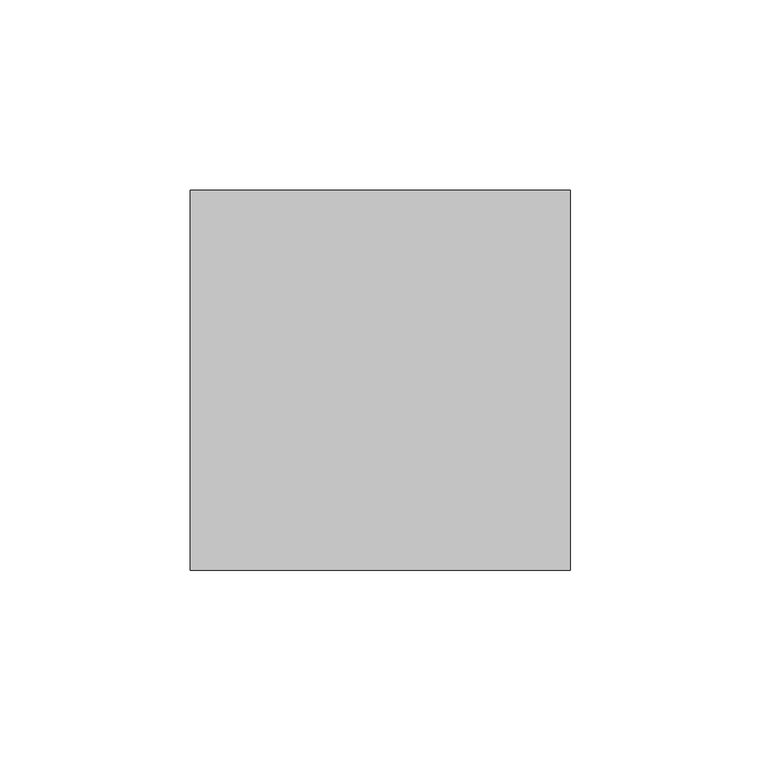
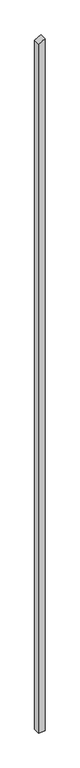
"""IFC4 building model written with IfcOpenShell, lengths in millimetres: column geometry, Holzstütze 158756 : Holzstütze 158756."""

import ifcopenshell
import ifcopenshell.guid

model = None  # the IFC model being written
_history = None  # IfcOwnerHistory: only IFC2X3 demands one
_inside = {}  # id of a spatial element -> (the spatial element, [elements in it])
_under = {}  # id of a project, library or spatial element -> (it, [spatial elements below it])
_declared = {}  # id of a project -> (the project, [libraries it declares])
_typed = {}  # id of a type object -> (the type object, [elements of that type])
_made_of = {}  # id of a material, layer set ... -> (it, [elements and type objects made of it])


def new_model(schema):
    """Start an empty IFC model of exactly this schema.

    Asked for "IFC4X3", IfcOpenShell would pick the latest addendum, in which some entities
    have other attributes; the version numbers below select the first issue.
    IFC2X3 requires an IfcOwnerHistory on every rooted entity: one is made here for all.
    """
    global model, _history
    if schema == "IFC4X3":
        model = ifcopenshell.file(schema_version=(4, 3, 0, 0))
    else:
        model = ifcopenshell.file(schema=schema)
    _inside.clear()
    _under.clear()
    _declared.clear()
    _typed.clear()
    _made_of.clear()
    _history = None
    if model.schema == "IFC2X3":
        org = make("IfcOrganization", Name="unknown")
        user = make(
            "IfcPersonAndOrganization",
            ThePerson=make("IfcPerson", FamilyName="unknown"),
            TheOrganization=org,
        )
        app = make(
            "IfcApplication",
            ApplicationDeveloper=org,
            Version="unknown",
            ApplicationFullName="unknown",
            ApplicationIdentifier="unknown",
        )
        _history = make(
            "IfcOwnerHistory",
            OwningUser=user,
            OwningApplication=app,
            ChangeAction="ADDED",
            CreationDate=0,
        )
    return model


def make(cls, **values):
    """One entity of the class cls with the attributes given. An attribute that is None is left unset."""
    return model.create_entity(
        cls, **{name: value for name, value in values.items() if value is not None}
    )


def rooted(cls, **values):
    """An entity with a GlobalId (a new one), such as an element, a storey or a relation."""
    return make(cls, GlobalId=ifcopenshell.guid.new(), OwnerHistory=_history, **values)


def si_unit(unit_type, name, prefix=None):
    """IfcSIUnit, for example si_unit("LENGTHUNIT", "METRE", prefix="MILLI")."""
    return make("IfcSIUnit", UnitType=unit_type, Prefix=prefix, Name=name)


def assignment(units):
    """IfcUnitAssignment: the units of a project."""
    return None if units is None else make("IfcUnitAssignment", Units=units)


def point(xyz):
    """IfcCartesianPoint."""
    return None if xyz is None else make("IfcCartesianPoint", Coordinates=xyz)


def direction(xyz):
    """IfcDirection."""
    return None if xyz is None else make("IfcDirection", DirectionRatios=xyz)


def frame(location, z_axis=None, x_axis=None):
    """IfcAxis2Placement3D, a coordinate frame: its origin and axes. An axis left out is left unset."""
    return make(
        "IfcAxis2Placement3D",
        Location=point(location),
        Axis=direction(z_axis),
        RefDirection=direction(x_axis),
    )


def origin():
    """The frame at (0, 0, 0) with its axes left unset."""
    return frame((0.0, 0.0, 0.0))


def place(relative_to, where):
    """IfcLocalPlacement: puts the frame where relative to a parent placement (None: the world)."""
    return make(
        "IfcLocalPlacement", PlacementRelTo=relative_to, RelativePlacement=where
    )


def context(
    kind, dimensions, precision=None, world=None, true_north=None, identifier=None
):
    """IfcGeometricRepresentationContext, for example the 3D "Model" context."""
    return make(
        "IfcGeometricRepresentationContext",
        ContextIdentifier=identifier,
        ContextType=kind,
        CoordinateSpaceDimension=dimensions,
        Precision=precision,
        WorldCoordinateSystem=world,
        TrueNorth=true_north,
    )


def project(units=None, contexts=None):
    """IfcProject with its units and contexts."""
    return rooted(
        "IfcProject",
        Name="project",
        RepresentationContexts=contexts,
        UnitsInContext=assignment(units),
    )


def spatial(cls, under=None, at=None, **own):
    """A site, building, storey or space (cls), placed at a placement, below another one or the project."""
    s = rooted(cls, ObjectPlacement=at, **own)
    if under is not None:
        _under.setdefault(under.id(), (under, []))[1].append(s)
    return s


def polyline(points):
    """IfcPolyline through the points."""
    return make("IfcPolyline", Points=[point(p) for p in points])


def outline(outer, holes=None, kind="AREA"):
    """IfcArbitraryClosedProfileDef: a profile drawn as a closed curve; with holes, ...WithVoids."""
    if holes is None:
        return make("IfcArbitraryClosedProfileDef", ProfileType=kind, OuterCurve=outer)
    return make(
        "IfcArbitraryProfileDefWithVoids",
        ProfileType=kind,
        OuterCurve=outer,
        InnerCurves=holes,
    )


def extrude(swept, where, along, depth):
    """IfcExtrudedAreaSolid: the profile swept, set in the frame where, extruded along a direction by depth."""
    return make(
        "IfcExtrudedAreaSolid",
        SweptArea=swept,
        Position=where,
        ExtrudedDirection=direction(along),
        Depth=depth,
    )


def shape(context_of_items, identifier, shape_type, items):
    """IfcShapeRepresentation: the items that make up one representation, for example the "Body"."""
    return make(
        "IfcShapeRepresentation",
        ContextOfItems=context_of_items,
        RepresentationIdentifier=identifier,
        RepresentationType=shape_type,
        Items=items,
    )


def source(mapping_origin, context_of_items, identifier, shape_type, items):
    """IfcRepresentationMap: a shape defined once, which mapped items show again and again."""
    return make(
        "IfcRepresentationMap",
        MappingOrigin=mapping_origin,
        MappedRepresentation=shape(context_of_items, identifier, shape_type, items),
    )


def transform(
    local_origin,
    x_axis=None,
    y_axis=None,
    z_axis=None,
    scale=None,
    scale2=None,
    scale3=None,
    uniform=True,
):
    """IfcCartesianTransformationOperator3D, or its non-uniform kind. x_axis, y_axis, z_axis: its Axis1, 2, 3."""
    if uniform:
        return make(
            "IfcCartesianTransformationOperator3D",
            Axis1=direction(x_axis),
            Axis2=direction(y_axis),
            LocalOrigin=point(local_origin),
            Scale=scale,
            Axis3=direction(z_axis),
        )
    return make(
        "IfcCartesianTransformationOperator3DnonUniform",
        Axis1=direction(x_axis),
        Axis2=direction(y_axis),
        LocalOrigin=point(local_origin),
        Scale=scale,
        Axis3=direction(z_axis),
        Scale2=scale2,
        Scale3=scale3,
    )


def mapped(mapping_source, mapping_target):
    """IfcMappedItem: shows the shape of a source again, moved by a transform."""
    return make(
        "IfcMappedItem", MappingSource=mapping_source, MappingTarget=mapping_target
    )


def made_of(thing, what):
    """Note that an element or type object is made of a material, layer set ...; save() writes the relation."""
    if what is not None:
        _made_of.setdefault(what.id(), (what, []))[1].append(thing)
    return thing


def element(
    cls,
    number,
    at=None,
    inside=None,
    cuts=None,
    type_object=None,
    material=None,
    context=None,
    identifier="Body",
    shape_type=None,
    held_by="IfcProductDefinitionShape",
    body=None,
    shapes=None,
    **own,
):
    """One element of the class cls, such as IfcWall. Its Tag is "e" and its number.

    at: its placement. inside: the storey or other place that contains it. cuts: it is an
    opening in that element (IfcRelVoidsElement). A single representation is given by context,
    identifier, shape_type and body (its items); several are given by shapes. held_by: the class
    of the entity that holds the representations. save() writes the other relations.
    """
    e = rooted(cls, Tag="e%d" % number, ObjectPlacement=at, **own)
    if body is not None:
        shapes = [shape(context, identifier, shape_type, body)]
    if shapes is not None:
        e.Representation = make(held_by, Representations=shapes)
    if inside is not None:
        _inside.setdefault(inside.id(), (inside, []))[1].append(e)
    if cuts is not None:
        rooted(
            "IfcRelVoidsElement", RelatingBuildingElement=cuts, RelatedOpeningElement=e
        )
    if type_object is not None:
        _typed.setdefault(type_object.id(), (type_object, []))[1].append(e)
    return made_of(e, material)


def aggregate(whole, parts):
    """IfcRelAggregates: a whole, such as a stair, and the parts it consists of."""
    return rooted("IfcRelAggregates", RelatingObject=whole, RelatedObjects=parts)


def save(model, path):
    """Write the relations noted so far, then the file.

    IfcRelAggregates (storeys below a building ...), IfcRelContainedInSpatialStructure (elements
    in a storey), IfcRelDefinesByType, IfcRelAssociatesMaterial and IfcRelDeclares: one each for
    every whole, place, type object, material and project.
    """
    for whole, parts in _under.values():
        aggregate(whole, parts)
    for where, things in _inside.values():
        rooted(
            "IfcRelContainedInSpatialStructure",
            RelatedElements=things,
            RelatingStructure=where,
        )
    for kind, things in _typed.values():
        rooted("IfcRelDefinesByType", RelatedObjects=things, RelatingType=kind)
    for what, things in _made_of.values():
        rooted("IfcRelAssociatesMaterial", RelatedObjects=things, RelatingMaterial=what)
    for by, libraries in _declared.values():
        rooted("IfcRelDeclares", RelatingContext=by, RelatedDefinitions=libraries)
    model.write(path)


def column_c7102fa8(model_context):
    return source(origin(), model_context, "Body", "SweptSolid", [
        extrude(outline(polyline([(-500.0, 165627.7593015), (-500.0, 165727.7593015), (10641.011365, 165727.7593015), (10590.0588201, 165627.7593015), (-500.0, 165627.7593015)])), frame((0.0, 47884.7962965, 0.0), z_axis=(0.0, 1.0, 0.0), x_axis=(0.0, 0.0, 1.0)), (0.0, 0.0, 1.0), 100.0),
    ])


if __name__ == "__main__":
    model = new_model("IFC4")
    model_context = context("Model", 3, world=origin())
    ifc_project = project(units=[si_unit("LENGTHUNIT", "METRE", prefix="MILLI")], contexts=[model_context])
    site = spatial("IfcSite", under=ifc_project)
    building = spatial("IfcBuilding", under=site)
    placement = place(None, origin())
    column_shape = column_c7102fa8(model_context)
    element("IfcColumn", 1, ObjectType="Holzstütze 158756 : Holzstütze 158756", at=placement, inside=building, context=model_context, shape_type="MappedRepresentation", body=[
        mapped(column_shape, transform((0.0, 0.0, 0.0), x_axis=(1.0, 0.0, 0.0), y_axis=(0.0, 1.0, 0.0), z_axis=(0.0, 0.0, 1.0))),
    ])
    save(model, "model.ifc")

# Revit data of these elements
# Type "Holzstütze 158756 : Holzstütze 158756"
#   Abrechnungsart = "m"
#   Allright_Bauteil_ID = "0152St 0000143526"
#   Bezeichnung = "Holzstütze"
#   Codetext = "ST-HOLZ\\"
#   Gewerk = "Zimmer- und Holzbauarbeiten"
#   Material = "Holz"
#   Objektname = "Stütze"
#   NameOverride = "Holzstütze"
#   Reference = "Holzstütze"
#   Status = "NEW"
#   ThermalTransmittance = 0.0000 BTU/(h·ft²·°F)
#   Roll = 0.00°
#   Slope = 0.00°
#   2D Interaktion = yes
#   IsExternal = yes
#   LoadBearing = yes
# Element 1 (IfcColumn, "Holzstütze 158756 : Holzstütze 158756")
#   Materials on its faces: "holzschalung"
# Materials
#   "holzschalung": class "Unassigned", colour RGB 128 128 128, transparency 0
